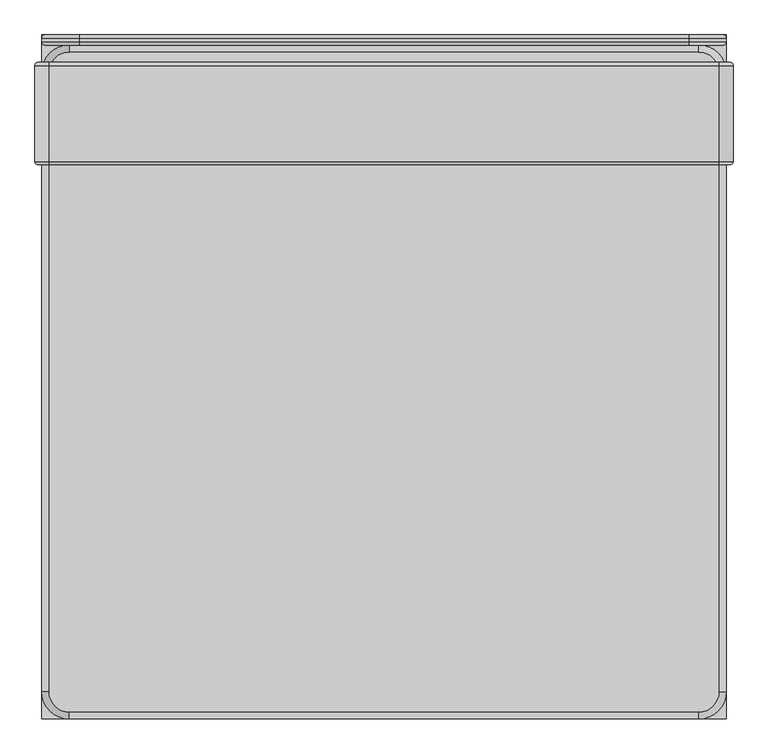
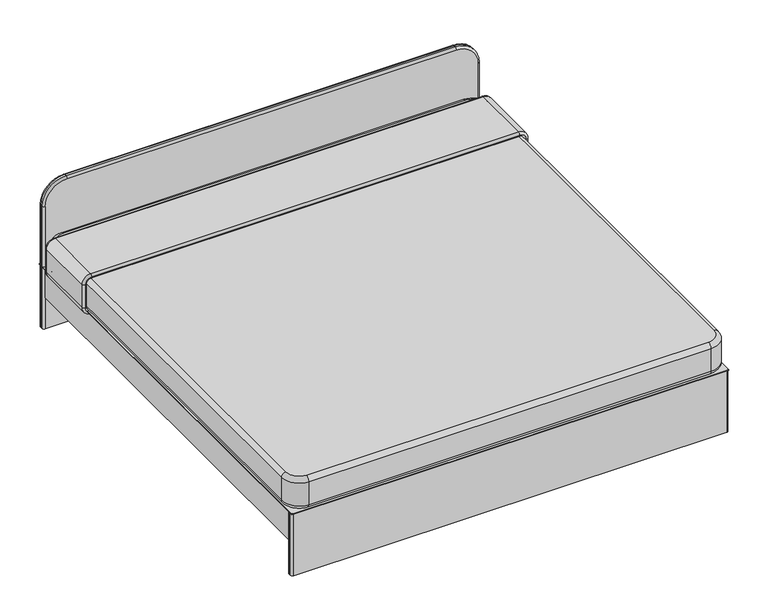
"""IFC4 building model written with IfcOpenShell, lengths in millimetres: furniture geometry, ベッド : 2000 x 2000 mm キング."""

from ifc_helpers import new_model, si_unit, point, frame, frame_2d, origin, origin_with_axes, place, context, project, spatial, polyline, circle_curve, ellipse_curve, trimmed, segment, composite_curve, outline, extrude, source, transform, mapped, element, save
from ifc_brep_helpers import plane_surface, cylinder_surface, revolved_surface, advanced_brep


def furniture_9038af62(model_context):
    return source(origin(), model_context, "Body", "SolidModel", [
        advanced_brep(
        [(1000.0, 960.0, 430.0), (1000.0, 680.0, 430.0), (980.0, 680.0, 450.0), (980.0, 960.0, 450.0), (1010.0, 970.0, 430.0), (980.0, 970.0, 460.0), (1020.0, 960.0, 430.0), (980.0, 960.0, 470.0), (1020.0, 680.0, 430.0), (980.0, 680.0, 470.0), (1010.0, 670.0, 430.0), (980.0, 670.0, 460.0), (1000.0, 960.0, 320.0), (1000.0, 680.0, 320.0), (1010.0, 970.0, 320.0), (1020.0, 960.0, 320.0), (1020.0, 680.0, 320.0), (1010.0, 670.0, 320.0), (980.0, 960.0, 300.0), (980.0, 680.0, 300.0), (980.0, 970.0, 290.0), (980.0, 960.0, 280.0), (980.0, 680.0, 280.0), (980.0, 670.0, 290.0), (-980.0, 960.0, 300.0), (-980.0, 680.0, 300.0), (-980.0, 970.0, 290.0), (-980.0, 960.0, 280.0), (-980.0, 680.0, 280.0), (-980.0, 670.0, 290.0), (-1000.0, 960.0, 320.0), (-1000.0, 680.0, 320.0), (-1010.0, 970.0, 320.0), (-1020.0, 960.0, 320.0), (-1020.0, 680.0, 320.0), (-1010.0, 670.0, 320.0), (-1000.0, 960.0, 430.0), (-1000.0, 680.0, 430.0), (-1010.0, 970.0, 430.0), (-1020.0, 960.0, 430.0), (-1020.0, 680.0, 430.0), (-1010.0, 670.0, 430.0), (-980.0, 960.0, 450.0), (-980.0, 680.0, 450.0), (-980.0, 970.0, 460.0), (-980.0, 960.0, 470.0), (-980.0, 680.0, 470.0), (-980.0, 670.0, 460.0)],
        [
            (0, 1),
            (1, 2, circle_curve(frame((980.0, 680.0, 430.0), z_axis=(0.0, -1.0, 0.0), x_axis=(0.0, 0.0, 1.0)), 20.0)),
            (2, 3),
            (3, 0, circle_curve(frame((980.0, 960.0, 430.0), z_axis=(0.0, 1.0, 0.0), x_axis=(0.0, 0.0, 1.0)), 20.0)),
            (4, 0, circle_curve(frame((1010.0, 960.0, 430.0), z_axis=(0.0, 0.0, 1.0), x_axis=(1.0, 0.0, 0.0)), 10.0)),
            (3, 5, circle_curve(frame((980.0, 960.0, 460.0), z_axis=(1.0, 0.0, 0.0), x_axis=(0.0, 0.0, 1.0)), 10.0)),
            (5, 4, circle_curve(frame((980.0, 970.0, 430.0), z_axis=(0.0, 1.0, 0.0), x_axis=(0.0, 0.0, 1.0)), 30.0)),
            (6, 4, circle_curve(frame((1010.0, 960.0, 430.0), z_axis=(0.0, 0.0, 1.0), x_axis=(1.0, 0.0, 0.0)), 10.0)),
            (5, 7, circle_curve(frame((980.0, 960.0, 460.0), z_axis=(1.0, 0.0, 0.0), x_axis=(0.0, 0.0, 1.0)), 10.0)),
            (7, 6, circle_curve(frame((980.0, 960.0, 430.0), z_axis=(0.0, 1.0, 0.0), x_axis=(0.0, 0.0, 1.0)), 40.0)),
            (8, 6),
            (7, 9),
            (9, 8, circle_curve(frame((980.0, 680.0, 430.0), z_axis=(0.0, 1.0, 0.0), x_axis=(0.0, 0.0, 1.0)), 40.0)),
            (10, 8, circle_curve(frame((1010.0, 680.0, 430.0), z_axis=(0.0, 0.0, 1.0), x_axis=(1.0, 0.0, 0.0)), 10.0)),
            (9, 11, circle_curve(frame((980.0, 680.0, 460.0), z_axis=(1.0, 0.0, 0.0), x_axis=(0.0, 0.0, 1.0)), 10.0)),
            (11, 10, circle_curve(frame((980.0, 670.0, 430.0), z_axis=(0.0, 1.0, 0.0), x_axis=(0.0, 0.0, 1.0)), 30.0)),
            (1, 10, circle_curve(frame((1010.0, 680.0, 430.0), z_axis=(0.0, 0.0, 1.0), x_axis=(1.0, 0.0, 0.0)), 10.0)),
            (11, 2, circle_curve(frame((980.0, 680.0, 460.0), z_axis=(1.0, 0.0, 0.0), x_axis=(0.0, 0.0, 1.0)), 10.0)),
            (0, 12),
            (12, 13),
            (13, 1),
            (4, 14),
            (14, 12, circle_curve(frame((1010.0, 960.0, 320.0), z_axis=(0.0, 0.0, 1.0), x_axis=(1.0, 0.0, 0.0)), 10.0)),
            (6, 15),
            (15, 14, circle_curve(frame((1010.0, 960.0, 320.0), z_axis=(0.0, 0.0, 1.0), x_axis=(1.0, 0.0, 0.0)), 10.0)),
            (8, 16),
            (16, 15),
            (10, 17),
            (17, 16, circle_curve(frame((1010.0, 680.0, 320.0), z_axis=(0.0, 0.0, 1.0), x_axis=(1.0, 0.0, 0.0)), 10.0)),
            (13, 17, circle_curve(frame((1010.0, 680.0, 320.0), z_axis=(0.0, 0.0, 1.0), x_axis=(1.0, 0.0, 0.0)), 10.0)),
            (18, 19),
            (19, 13, circle_curve(frame((980.0, 680.0, 320.0), z_axis=(0.0, -1.0, 0.0), x_axis=(1.0, 0.0, 0.0)), 20.0)),
            (12, 18, circle_curve(frame((980.0, 960.0, 320.0), z_axis=(0.0, 1.0, 0.0), x_axis=(1.0, 0.0, 0.0)), 20.0)),
            (20, 18, circle_curve(frame((980.0, 960.0, 290.0), z_axis=(1.0, 0.0, 0.0), x_axis=(0.0, 0.0, -1.0)), 10.0)),
            (14, 20, circle_curve(frame((980.0, 970.0, 320.0), z_axis=(0.0, 1.0, 0.0), x_axis=(1.0, 0.0, 0.0)), 30.0)),
            (21, 20, circle_curve(frame((980.0, 960.0, 290.0), z_axis=(1.0, 0.0, 0.0), x_axis=(0.0, 0.0, -1.0)), 10.0)),
            (15, 21, circle_curve(frame((980.0, 960.0, 320.0), z_axis=(0.0, 1.0, 0.0), x_axis=(1.0, 0.0, 0.0)), 40.0)),
            (22, 21),
            (16, 22, circle_curve(frame((980.0, 680.0, 320.0), z_axis=(0.0, 1.0, 0.0), x_axis=(1.0, 0.0, 0.0)), 40.0)),
            (23, 22, circle_curve(frame((980.0, 680.0, 290.0), z_axis=(1.0, 0.0, 0.0), x_axis=(0.0, 0.0, -1.0)), 10.0)),
            (17, 23, circle_curve(frame((980.0, 670.0, 320.0), z_axis=(0.0, 1.0, 0.0), x_axis=(1.0, 0.0, 0.0)), 30.0)),
            (19, 23, circle_curve(frame((980.0, 680.0, 290.0), z_axis=(1.0, 0.0, 0.0), x_axis=(0.0, 0.0, -1.0)), 10.0)),
            (18, 24),
            (24, 25),
            (25, 19),
            (20, 26),
            (26, 24, circle_curve(frame((-980.0, 960.0, 290.0), z_axis=(1.0, 0.0, 0.0), x_axis=(0.0, 0.0, -1.0)), 10.0)),
            (21, 27),
            (27, 26, circle_curve(frame((-980.0, 960.0, 290.0), z_axis=(1.0, 0.0, 0.0), x_axis=(0.0, 0.0, -1.0)), 10.0)),
            (22, 28),
            (28, 27),
            (23, 29),
            (29, 28, circle_curve(frame((-980.0, 680.0, 290.0), z_axis=(1.0, 0.0, 0.0), x_axis=(0.0, 0.0, -1.0)), 10.0)),
            (25, 29, circle_curve(frame((-980.0, 680.0, 290.0), z_axis=(1.0, 0.0, 0.0), x_axis=(0.0, 0.0, -1.0)), 10.0)),
            (30, 31),
            (31, 25, circle_curve(frame((-980.0, 680.0, 320.0), z_axis=(0.0, -1.0, 0.0), x_axis=(0.0, 0.0, -1.0)), 20.0)),
            (24, 30, circle_curve(frame((-980.0, 960.0, 320.0), z_axis=(0.0, 1.0, 0.0), x_axis=(0.0, 0.0, -1.0)), 20.0)),
            (32, 30, circle_curve(frame((-1010.0, 960.0, 320.0), z_axis=(0.0, 0.0, -1.0), x_axis=(-1.0, 0.0, 0.0)), 10.0)),
            (26, 32, circle_curve(frame((-980.0, 970.0, 320.0), z_axis=(0.0, 1.0, 0.0), x_axis=(0.0, 0.0, -1.0)), 30.0)),
            (33, 32, circle_curve(frame((-1010.0, 960.0, 320.0), z_axis=(0.0, 0.0, -1.0), x_axis=(-1.0, 0.0, 0.0)), 10.0)),
            (27, 33, circle_curve(frame((-980.0, 960.0, 320.0), z_axis=(0.0, 1.0, 0.0), x_axis=(0.0, 0.0, -1.0)), 40.0)),
            (34, 33),
            (28, 34, circle_curve(frame((-980.0, 680.0, 320.0), z_axis=(0.0, 1.0, 0.0), x_axis=(0.0, 0.0, -1.0)), 40.0)),
            (35, 34, circle_curve(frame((-1010.0, 680.0, 320.0), z_axis=(0.0, 0.0, -1.0), x_axis=(-1.0, 0.0, 0.0)), 10.0)),
            (29, 35, circle_curve(frame((-980.0, 670.0, 320.0), z_axis=(0.0, 1.0, 0.0), x_axis=(0.0, 0.0, -1.0)), 30.0)),
            (31, 35, circle_curve(frame((-1010.0, 680.0, 320.0), z_axis=(0.0, 0.0, -1.0), x_axis=(-1.0, 0.0, 0.0)), 10.0)),
            (30, 36),
            (36, 37),
            (37, 31),
            (32, 38),
            (38, 36, circle_curve(frame((-1010.0, 960.0, 430.0), z_axis=(0.0, 0.0, -1.0), x_axis=(-1.0, 0.0, 0.0)), 10.0)),
            (33, 39),
            (39, 38, circle_curve(frame((-1010.0, 960.0, 430.0), z_axis=(0.0, 0.0, -1.0), x_axis=(-1.0, 0.0, 0.0)), 10.0)),
            (34, 40),
            (40, 39),
            (35, 41),
            (41, 40, circle_curve(frame((-1010.0, 680.0, 430.0), z_axis=(0.0, 0.0, -1.0), x_axis=(-1.0, 0.0, 0.0)), 10.0)),
            (37, 41, circle_curve(frame((-1010.0, 680.0, 430.0), z_axis=(0.0, 0.0, -1.0), x_axis=(-1.0, 0.0, 0.0)), 10.0)),
            (42, 43),
            (43, 37, circle_curve(frame((-980.0, 680.0, 430.0), z_axis=(0.0, -1.0, 0.0), x_axis=(-1.0, 0.0, 0.0)), 20.0)),
            (36, 42, circle_curve(frame((-980.0, 960.0, 430.0), z_axis=(0.0, 1.0, 0.0), x_axis=(-1.0, 0.0, 0.0)), 20.0)),
            (44, 42, circle_curve(frame((-980.0, 960.0, 460.0), z_axis=(-1.0, 0.0, 0.0), x_axis=(0.0, 0.0, 1.0)), 10.0)),
            (38, 44, circle_curve(frame((-980.0, 970.0, 430.0), z_axis=(0.0, 1.0, 0.0), x_axis=(-1.0, 0.0, 0.0)), 30.0)),
            (45, 44, circle_curve(frame((-980.0, 960.0, 460.0), z_axis=(-1.0, 0.0, 0.0), x_axis=(0.0, 0.0, 1.0)), 10.0)),
            (39, 45, circle_curve(frame((-980.0, 960.0, 430.0), z_axis=(0.0, 1.0, 0.0), x_axis=(-1.0, 0.0, 0.0)), 40.0)),
            (46, 45),
            (40, 46, circle_curve(frame((-980.0, 680.0, 430.0), z_axis=(0.0, 1.0, 0.0), x_axis=(-1.0, 0.0, 0.0)), 40.0)),
            (47, 46, circle_curve(frame((-980.0, 680.0, 460.0), z_axis=(-1.0, 0.0, 0.0), x_axis=(0.0, 0.0, 1.0)), 10.0)),
            (41, 47, circle_curve(frame((-980.0, 670.0, 430.0), z_axis=(0.0, 1.0, 0.0), x_axis=(-1.0, 0.0, 0.0)), 30.0)),
            (43, 47, circle_curve(frame((-980.0, 680.0, 460.0), z_axis=(-1.0, 0.0, 0.0), x_axis=(0.0, 0.0, 1.0)), 10.0)),
            (42, 3),
            (2, 43),
            (44, 5),
            (45, 7),
            (46, 9),
            (47, 11),
        ],
        [
            revolved_surface(polyline([(980.0, 680.0, 450.0), (980.0, 960.0, 450.0)]), (980.0, 970.0, 430.0), (0.0, -1.0, 0.0)),
            revolved_surface(trimmed(ellipse_curve(frame((980.0, 960.0, 460.0), z_axis=(1.0, 0.0, 0.0), x_axis=(0.0, 0.0, 1.0)), 10.0, 10.0), [point((980.0, 960.0, 450.0))], [point((980.0, 970.0, 460.0))], True, "CARTESIAN"), (980.0, 970.0, 430.0), (0.0, -1.0, 0.0)),
            revolved_surface(trimmed(ellipse_curve(frame((980.0, 960.0, 460.0), z_axis=(1.0, 0.0, 0.0), x_axis=(0.0, 0.0, 1.0)), 10.0, 10.0), [point((980.0, 970.0, 460.0))], [point((980.0, 960.0, 470.0))], True, "CARTESIAN"), (980.0, 970.0, 430.0), (0.0, -1.0, 0.0)),
            cylinder_surface(frame((980.0, 970.0, 430.0), z_axis=(0.0, -1.0, 0.0), x_axis=(0.0, 0.0, 1.0)), 40.0),
            revolved_surface(trimmed(ellipse_curve(frame((980.0, 680.0, 460.0), z_axis=(1.0, 0.0, 0.0), x_axis=(0.0, 0.0, 1.0)), 10.0, 10.0), [point((980.0, 680.0, 470.0))], [point((980.0, 670.0, 460.0))], True, "CARTESIAN"), (980.0, 970.0, 430.0), (0.0, -1.0, 0.0)),
            revolved_surface(trimmed(ellipse_curve(frame((980.0, 680.0, 460.0), z_axis=(1.0, 0.0, 0.0), x_axis=(0.0, 0.0, 1.0)), 10.0, 10.0), [point((980.0, 670.0, 460.0))], [point((980.0, 680.0, 450.0))], True, "CARTESIAN"), (980.0, 970.0, 430.0), (0.0, -1.0, 0.0)),
            plane_surface(frame((1000.0, 680.0, 430.0), z_axis=(-1.0, 0.0, 0.0), x_axis=(0.0, 0.0, -1.0))),
            cylinder_surface(frame((1010.0, 960.0, 430.0), z_axis=(0.0, 0.0, 1.0), x_axis=(1.0, 0.0, 0.0)), 10.0),
            plane_surface(frame((1020.0, 960.0, 430.0), z_axis=(1.0, 0.0, 0.0), x_axis=(0.0, 0.0, -1.0))),
            cylinder_surface(frame((1010.0, 680.0, 430.0), z_axis=(0.0, 0.0, 1.0), x_axis=(1.0, 0.0, 0.0)), 10.0),
            revolved_surface(polyline([(1000.0, 680.0, 320.0), (1000.0, 960.0, 320.0)]), (980.0, 970.0, 320.0), (0.0, -1.0, 0.0)),
            revolved_surface(trimmed(ellipse_curve(frame((1010.0, 960.0, 320.0), z_axis=(0.0, 0.0, -1.0), x_axis=(1.0, 0.0, 0.0)), 10.0, 10.0), [point((1000.0, 960.0, 320.0))], [point((1010.0, 970.0, 320.0))], True, "CARTESIAN"), (980.0, 970.0, 320.0), (0.0, -1.0, 0.0)),
            revolved_surface(trimmed(ellipse_curve(frame((1010.0, 960.0, 320.0), z_axis=(0.0, 0.0, -1.0), x_axis=(1.0, 0.0, 0.0)), 10.0, 10.0), [point((1010.0, 970.0, 320.0))], [point((1020.0, 960.0, 320.0))], True, "CARTESIAN"), (980.0, 970.0, 320.0), (0.0, -1.0, 0.0)),
            cylinder_surface(frame((980.0, 970.0, 320.0), z_axis=(0.0, -1.0, 0.0), x_axis=(1.0, 0.0, 0.0)), 40.0),
            revolved_surface(trimmed(ellipse_curve(frame((1010.0, 680.0, 320.0), z_axis=(0.0, 0.0, -1.0), x_axis=(1.0, 0.0, 0.0)), 10.0, 10.0), [point((1020.0, 680.0, 320.0))], [point((1010.0, 670.0, 320.0))], True, "CARTESIAN"), (980.0, 970.0, 320.0), (0.0, -1.0, 0.0)),
            revolved_surface(trimmed(ellipse_curve(frame((1010.0, 680.0, 320.0), z_axis=(0.0, 0.0, -1.0), x_axis=(1.0, 0.0, 0.0)), 10.0, 10.0), [point((1010.0, 670.0, 320.0))], [point((1000.0, 680.0, 320.0))], True, "CARTESIAN"), (980.0, 970.0, 320.0), (0.0, -1.0, 0.0)),
            plane_surface(frame((980.0, 680.0, 300.0), z_axis=(0.0, 0.0, 1.0), x_axis=(-1.0, 0.0, 0.0))),
            cylinder_surface(frame((980.0, 960.0, 290.0), z_axis=(1.0, 0.0, 0.0), x_axis=(0.0, 0.0, -1.0)), 10.0),
            plane_surface(frame((980.0, 960.0, 280.0), z_axis=(0.0, 0.0, -1.0), x_axis=(-1.0, 0.0, 0.0))),
            cylinder_surface(frame((980.0, 680.0, 290.0), z_axis=(1.0, 0.0, 0.0), x_axis=(0.0, 0.0, -1.0)), 10.0),
            revolved_surface(polyline([(-980.0, 680.0, 300.0), (-980.0, 960.0, 300.0)]), (-980.0, 970.0, 320.0), (0.0, -1.0, 0.0)),
            revolved_surface(trimmed(ellipse_curve(frame((-980.0, 960.0, 290.0), z_axis=(-1.0, 0.0, 0.0), x_axis=(0.0, 0.0, -1.0)), 10.0, 10.0), [point((-980.0, 960.0, 300.0))], [point((-980.0, 970.0, 290.0))], True, "CARTESIAN"), (-980.0, 970.0, 320.0), (0.0, -1.0, 0.0)),
            revolved_surface(trimmed(ellipse_curve(frame((-980.0, 960.0, 290.0), z_axis=(-1.0, 0.0, 0.0), x_axis=(0.0, 0.0, -1.0)), 10.0, 10.0), [point((-980.0, 970.0, 290.0))], [point((-980.0, 960.0, 280.0))], True, "CARTESIAN"), (-980.0, 970.0, 320.0), (0.0, -1.0, 0.0)),
            cylinder_surface(frame((-980.0, 970.0, 320.0), z_axis=(0.0, -1.0, 0.0), x_axis=(0.0, 0.0, -1.0)), 40.0),
            revolved_surface(trimmed(ellipse_curve(frame((-980.0, 680.0, 290.0), z_axis=(-1.0, 0.0, 0.0), x_axis=(0.0, 0.0, -1.0)), 10.0, 10.0), [point((-980.0, 680.0, 280.0))], [point((-980.0, 670.0, 290.0))], True, "CARTESIAN"), (-980.0, 970.0, 320.0), (0.0, -1.0, 0.0)),
            revolved_surface(trimmed(ellipse_curve(frame((-980.0, 680.0, 290.0), z_axis=(-1.0, 0.0, 0.0), x_axis=(0.0, 0.0, -1.0)), 10.0, 10.0), [point((-980.0, 670.0, 290.0))], [point((-980.0, 680.0, 300.0))], True, "CARTESIAN"), (-980.0, 970.0, 320.0), (0.0, -1.0, 0.0)),
            plane_surface(frame((-1000.0, 680.0, 320.0), z_axis=(1.0, 0.0, 0.0), x_axis=(0.0, 0.0, 1.0))),
            cylinder_surface(frame((-1010.0, 960.0, 320.0), z_axis=(0.0, 0.0, -1.0), x_axis=(-1.0, 0.0, 0.0)), 10.0),
            plane_surface(frame((-1020.0, 960.0, 320.0), z_axis=(-1.0, 0.0, 0.0), x_axis=(0.0, 0.0, 1.0))),
            cylinder_surface(frame((-1010.0, 680.0, 320.0), z_axis=(0.0, 0.0, -1.0), x_axis=(-1.0, 0.0, 0.0)), 10.0),
            revolved_surface(polyline([(-1000.0, 680.0, 430.0), (-1000.0, 960.0, 430.0)]), (-980.0, 970.0, 430.0), (0.0, -1.0, 0.0)),
            revolved_surface(trimmed(ellipse_curve(frame((-1010.0, 960.0, 430.0), z_axis=(0.0, 0.0, 1.0), x_axis=(-1.0, 0.0, 0.0)), 10.0, 10.0), [point((-1000.0, 960.0, 430.0))], [point((-1010.0, 970.0, 430.0))], True, "CARTESIAN"), (-980.0, 970.0, 430.0), (0.0, -1.0, 0.0)),
            revolved_surface(trimmed(ellipse_curve(frame((-1010.0, 960.0, 430.0), z_axis=(0.0, 0.0, 1.0), x_axis=(-1.0, 0.0, 0.0)), 10.0, 10.0), [point((-1010.0, 970.0, 430.0))], [point((-1020.0, 960.0, 430.0))], True, "CARTESIAN"), (-980.0, 970.0, 430.0), (0.0, -1.0, 0.0)),
            cylinder_surface(frame((-980.0, 970.0, 430.0), z_axis=(0.0, -1.0, 0.0), x_axis=(-1.0, 0.0, 0.0)), 40.0),
            revolved_surface(trimmed(ellipse_curve(frame((-1010.0, 680.0, 430.0), z_axis=(0.0, 0.0, 1.0), x_axis=(-1.0, 0.0, 0.0)), 10.0, 10.0), [point((-1020.0, 680.0, 430.0))], [point((-1010.0, 670.0, 430.0))], True, "CARTESIAN"), (-980.0, 970.0, 430.0), (0.0, -1.0, 0.0)),
            revolved_surface(trimmed(ellipse_curve(frame((-1010.0, 680.0, 430.0), z_axis=(0.0, 0.0, 1.0), x_axis=(-1.0, 0.0, 0.0)), 10.0, 10.0), [point((-1010.0, 670.0, 430.0))], [point((-1000.0, 680.0, 430.0))], True, "CARTESIAN"), (-980.0, 970.0, 430.0), (0.0, -1.0, 0.0)),
            plane_surface(frame((-980.0, 680.0, 450.0), z_axis=(0.0, 0.0, -1.0), x_axis=(1.0, 0.0, 0.0))),
            cylinder_surface(frame((-980.0, 960.0, 460.0), z_axis=(-1.0, 0.0, 0.0), x_axis=(0.0, 0.0, 1.0)), 10.0),
            plane_surface(frame((-980.0, 960.0, 470.0), z_axis=(0.0, 0.0, 1.0), x_axis=(1.0, 0.0, 0.0))),
            cylinder_surface(frame((-980.0, 680.0, 460.0), z_axis=(-1.0, 0.0, 0.0), x_axis=(0.0, 0.0, 1.0)), 10.0),
        ],
        [
            (0, [[1, 2, 3, 4]]),
            (1, [[5, -4, 6, 7]]),
            (2, [[8, -7, 9, 10]]),
            (3, [[11, -10, 12, 13]]),
            (4, [[14, -13, 15, 16]]),
            (5, [[17, -16, 18, -2]]),
            (6, [[19, 20, 21, -1]]),
            (7, [[22, 23, -19, -5]]),
            (7, [[24, 25, -22, -8]]),
            (8, [[26, 27, -24, -11]]),
            (9, [[28, 29, -26, -14]]),
            (9, [[-21, 30, -28, -17]]),
            (10, [[31, 32, -20, 33]]),
            (11, [[34, -33, -23, 35]]),
            (12, [[36, -35, -25, 37]]),
            (13, [[38, -37, -27, 39]]),
            (14, [[40, -39, -29, 41]]),
            (15, [[42, -41, -30, -32]]),
            (16, [[43, 44, 45, -31]]),
            (17, [[46, 47, -43, -34]]),
            (17, [[48, 49, -46, -36]]),
            (18, [[50, 51, -48, -38]]),
            (19, [[52, 53, -50, -40]]),
            (19, [[-45, 54, -52, -42]]),
            (20, [[55, 56, -44, 57]]),
            (21, [[58, -57, -47, 59]]),
            (22, [[60, -59, -49, 61]]),
            (23, [[62, -61, -51, 63]]),
            (24, [[64, -63, -53, 65]]),
            (25, [[66, -65, -54, -56]]),
            (26, [[67, 68, 69, -55]]),
            (27, [[70, 71, -67, -58]]),
            (27, [[72, 73, -70, -60]]),
            (28, [[74, 75, -72, -62]]),
            (29, [[76, 77, -74, -64]]),
            (29, [[-69, 78, -76, -66]]),
            (30, [[79, 80, -68, 81]]),
            (31, [[82, -81, -71, 83]]),
            (32, [[84, -83, -73, 85]]),
            (33, [[86, -85, -75, 87]]),
            (34, [[88, -87, -77, 89]]),
            (35, [[90, -89, -78, -80]]),
            (36, [[91, -3, 92, -79]]),
            (37, [[93, -6, -91, -82]]),
            (37, [[94, -9, -93, -84]]),
            (38, [[95, -12, -94, -86]]),
            (39, [[96, -15, -95, -88]]),
            (39, [[-92, -18, -96, -90]]),
        ],
    ),
        extrude(outline(polyline([(1000.0, 1050.0), (1000.0, -950.0), (-1000.0, -950.0), (-1000.0, 1050.0), (1000.0, 1050.0)])), frame((0.0, 0.0, 298.0), z_axis=(0.0, 0.0, 1.0), x_axis=(1.0, 0.0, 0.0)), (0.0, 0.0, 1.0), 2.0),
        advanced_brep(
        [(1000.0, 940.0, 320.0), (980.0, 940.0, 300.0), (920.0, 1000.0, 300.0), (920.0, 1020.0, 320.0), (920.0, 1020.0, 430.0), (1000.0, 940.0, 430.0), (920.0, 1000.0, 450.0), (980.0, 940.0, 450.0), (1000.0, -870.0, 320.0), (980.0, -870.0, 300.0), (1000.0, -870.0, 430.0), (980.0, -870.0, 450.0), (920.0, -950.0, 320.0), (920.0, -930.0, 300.0), (920.0, -950.0, 430.0), (920.0, -930.0, 450.0), (-920.0, -950.0, 320.0), (-920.0, -930.0, 300.0), (-920.0, -950.0, 430.0), (-920.0, -930.0, 450.0), (-1000.0, -870.0, 320.0), (-980.0, -870.0, 300.0), (-1000.0, -870.0, 430.0), (-980.0, -870.0, 450.0), (-1000.0, 940.0, 320.0), (-980.0, 940.0, 300.0), (-1000.0, 940.0, 430.0), (-980.0, 940.0, 450.0), (-920.0, 1020.0, 320.0), (-920.0, 1000.0, 300.0), (-920.0, 1020.0, 430.0), (-920.0, 1000.0, 450.0)],
        [
            (0, 1, circle_curve(frame((980.0, 940.0, 320.0), z_axis=(0.0, 1.0, 0.0), x_axis=(-1.0, 0.0, 0.0)), 20.0)),
            (1, 2, circle_curve(frame((920.0, 940.0, 300.0), z_axis=(0.0, 0.0, 1.0), x_axis=(0.0, 1.0, 0.0)), 60.0)),
            (2, 3, circle_curve(frame((920.0, 1000.0, 320.0), z_axis=(1.0, 0.0, 0.0), x_axis=(0.0, -1.0, 0.0)), 20.0)),
            (3, 0, circle_curve(frame((920.0, 940.0, 320.0), z_axis=(0.0, 0.0, -1.0), x_axis=(0.0, 1.0, 0.0)), 80.0)),
            (3, 4),
            (4, 5, circle_curve(frame((920.0, 940.0, 430.0), z_axis=(0.0, 0.0, -1.0), x_axis=(0.0, 1.0, 0.0)), 80.0)),
            (5, 0),
            (4, 6, circle_curve(frame((920.0, 1000.0, 430.0), z_axis=(1.0, 0.0, 0.0), x_axis=(0.0, -1.0, 0.0)), 20.0)),
            (6, 7, circle_curve(frame((920.0, 940.0, 450.0), z_axis=(0.0, 0.0, -1.0), x_axis=(0.0, 1.0, 0.0)), 60.0)),
            (7, 5, circle_curve(frame((980.0, 940.0, 430.0), z_axis=(0.0, 1.0, 0.0), x_axis=(-1.0, 0.0, 0.0)), 20.0)),
            (0, 8),
            (8, 9, circle_curve(frame((980.0, -870.0, 320.0), z_axis=(0.0, 1.0, 0.0), x_axis=(-1.0, 0.0, 0.0)), 20.0)),
            (9, 1),
            (5, 10),
            (10, 8),
            (7, 11),
            (11, 10, circle_curve(frame((980.0, -870.0, 430.0), z_axis=(0.0, 1.0, 0.0), x_axis=(-1.0, 0.0, 0.0)), 20.0)),
            (8, 12, circle_curve(frame((920.0, -870.0, 320.0), z_axis=(0.0, 0.0, -1.0), x_axis=(1.0, 0.0, 0.0)), 80.0)),
            (12, 13, circle_curve(frame((920.0, -930.0, 320.0), z_axis=(1.0, 0.0, 0.0), x_axis=(0.0, 1.0, 0.0)), 20.0)),
            (13, 9, circle_curve(frame((920.0, -870.0, 300.0), z_axis=(0.0, 0.0, 1.0), x_axis=(1.0, 0.0, 0.0)), 60.0)),
            (10, 14, circle_curve(frame((920.0, -870.0, 430.0), z_axis=(0.0, 0.0, -1.0), x_axis=(1.0, 0.0, 0.0)), 80.0)),
            (14, 12),
            (11, 15, circle_curve(frame((920.0, -870.0, 450.0), z_axis=(0.0, 0.0, -1.0), x_axis=(1.0, 0.0, 0.0)), 60.0)),
            (15, 14, circle_curve(frame((920.0, -930.0, 430.0), z_axis=(1.0, 0.0, 0.0), x_axis=(0.0, 1.0, 0.0)), 20.0)),
            (12, 16),
            (16, 17, circle_curve(frame((-920.0, -930.0, 320.0), z_axis=(1.0, 0.0, 0.0), x_axis=(0.0, 1.0, 0.0)), 20.0)),
            (17, 13),
            (14, 18),
            (18, 16),
            (15, 19),
            (19, 18, circle_curve(frame((-920.0, -930.0, 430.0), z_axis=(1.0, 0.0, 0.0), x_axis=(0.0, 1.0, 0.0)), 20.0)),
            (16, 20, circle_curve(frame((-920.0, -870.0, 320.0), z_axis=(0.0, 0.0, -1.0), x_axis=(0.0, -1.0, 0.0)), 80.0)),
            (20, 21, circle_curve(frame((-980.0, -870.0, 320.0), z_axis=(0.0, -1.0, 0.0), x_axis=(1.0, 0.0, 0.0)), 20.0)),
            (21, 17, circle_curve(frame((-920.0, -870.0, 300.0), z_axis=(0.0, 0.0, 1.0), x_axis=(0.0, -1.0, 0.0)), 60.0)),
            (18, 22, circle_curve(frame((-920.0, -870.0, 430.0), z_axis=(0.0, 0.0, -1.0), x_axis=(0.0, -1.0, 0.0)), 80.0)),
            (22, 20),
            (19, 23, circle_curve(frame((-920.0, -870.0, 450.0), z_axis=(0.0, 0.0, -1.0), x_axis=(0.0, -1.0, 0.0)), 60.0)),
            (23, 22, circle_curve(frame((-980.0, -870.0, 430.0), z_axis=(0.0, -1.0, 0.0), x_axis=(1.0, 0.0, 0.0)), 20.0)),
            (20, 24),
            (24, 25, circle_curve(frame((-980.0, 940.0, 320.0), z_axis=(0.0, -1.0, 0.0), x_axis=(1.0, 0.0, 0.0)), 20.0)),
            (25, 21),
            (22, 26),
            (26, 24),
            (23, 27),
            (27, 26, circle_curve(frame((-980.0, 940.0, 430.0), z_axis=(0.0, -1.0, 0.0), x_axis=(1.0, 0.0, 0.0)), 20.0)),
            (24, 28, circle_curve(frame((-920.0, 940.0, 320.0), z_axis=(0.0, 0.0, -1.0), x_axis=(-1.0, 0.0, 0.0)), 80.0)),
            (28, 29, circle_curve(frame((-920.0, 1000.0, 320.0), z_axis=(-1.0, 0.0, 0.0), x_axis=(0.0, -1.0, 0.0)), 20.0)),
            (29, 25, circle_curve(frame((-920.0, 940.0, 300.0), z_axis=(0.0, 0.0, 1.0), x_axis=(-1.0, 0.0, 0.0)), 60.0)),
            (26, 30, circle_curve(frame((-920.0, 940.0, 430.0), z_axis=(0.0, 0.0, -1.0), x_axis=(-1.0, 0.0, 0.0)), 80.0)),
            (30, 28),
            (27, 31, circle_curve(frame((-920.0, 940.0, 450.0), z_axis=(0.0, 0.0, -1.0), x_axis=(-1.0, 0.0, 0.0)), 60.0)),
            (31, 30, circle_curve(frame((-920.0, 1000.0, 430.0), z_axis=(-1.0, 0.0, 0.0), x_axis=(0.0, -1.0, 0.0)), 20.0)),
            (6, 31),
            (29, 2),
            (28, 3),
            (30, 4),
        ],
        [
            revolved_surface(trimmed(ellipse_curve(frame((920.0, 1000.0, 320.0), z_axis=(1.0, 0.0, 0.0), x_axis=(0.0, -1.0, 0.0)), 20.0, 20.0), [point((920.0, 1000.0, 300.0))], [point((920.0, 1020.0, 320.0))], True, "CARTESIAN"), (920.0, 940.0, 300.0), (0.0, 0.0, 1.0)),
            cylinder_surface(frame((920.0, 940.0, 300.0), z_axis=(0.0, 0.0, 1.0), x_axis=(0.0, 1.0, 0.0)), 80.0),
            revolved_surface(trimmed(ellipse_curve(frame((920.0, 1000.0, 430.0), z_axis=(1.0, 0.0, 0.0), x_axis=(0.0, -1.0, 0.0)), 20.0, 20.0), [point((920.0, 1020.0, 430.0))], [point((920.0, 1000.0, 450.0))], True, "CARTESIAN"), (920.0, 940.0, 300.0), (0.0, 0.0, 1.0)),
            cylinder_surface(frame((980.0, 940.0, 320.0), z_axis=(0.0, 1.0, 0.0), x_axis=(-1.0, 0.0, 0.0)), 20.0),
            plane_surface(frame((1000.0, 940.0, 320.0), z_axis=(1.0, 0.0, 0.0), x_axis=(0.0, -1.0, 0.0))),
            cylinder_surface(frame((980.0, 940.0, 430.0), z_axis=(0.0, 1.0, 0.0), x_axis=(-1.0, 0.0, 0.0)), 20.0),
            revolved_surface(trimmed(ellipse_curve(frame((980.0, -870.0, 320.0), z_axis=(0.0, -1.0, 0.0), x_axis=(-1.0, 0.0, 0.0)), 20.0, 20.0), [point((980.0, -870.0, 300.0))], [point((1000.0, -870.0, 320.0))], True, "CARTESIAN"), (920.0, -870.0, 300.0), (0.0, 0.0, 1.0)),
            cylinder_surface(frame((920.0, -870.0, 300.0), z_axis=(0.0, 0.0, 1.0), x_axis=(1.0, 0.0, 0.0)), 80.0),
            revolved_surface(trimmed(ellipse_curve(frame((980.0, -870.0, 430.0), z_axis=(0.0, -1.0, 0.0), x_axis=(-1.0, 0.0, 0.0)), 20.0, 20.0), [point((1000.0, -870.0, 430.0))], [point((980.0, -870.0, 450.0))], True, "CARTESIAN"), (920.0, -870.0, 300.0), (0.0, 0.0, 1.0)),
            cylinder_surface(frame((920.0, -930.0, 320.0), z_axis=(1.0, 0.0, 0.0), x_axis=(0.0, 1.0, 0.0)), 20.0),
            plane_surface(frame((920.0, -950.0, 320.0), z_axis=(0.0, -1.0, 0.0), x_axis=(-1.0, 0.0, 0.0))),
            cylinder_surface(frame((920.0, -930.0, 430.0), z_axis=(1.0, 0.0, 0.0), x_axis=(0.0, 1.0, 0.0)), 20.0),
            revolved_surface(trimmed(ellipse_curve(frame((-920.0, -930.0, 320.0), z_axis=(-1.0, 0.0, 0.0), x_axis=(0.0, 1.0, 0.0)), 20.0, 20.0), [point((-920.0, -930.0, 300.0))], [point((-920.0, -950.0, 320.0))], True, "CARTESIAN"), (-920.0, -870.0, 300.0), (0.0, 0.0, 1.0)),
            cylinder_surface(frame((-920.0, -870.0, 300.0), z_axis=(0.0, 0.0, 1.0), x_axis=(0.0, -1.0, 0.0)), 80.0),
            revolved_surface(trimmed(ellipse_curve(frame((-920.0, -930.0, 430.0), z_axis=(-1.0, 0.0, 0.0), x_axis=(0.0, 1.0, 0.0)), 20.0, 20.0), [point((-920.0, -950.0, 430.0))], [point((-920.0, -930.0, 450.0))], True, "CARTESIAN"), (-920.0, -870.0, 300.0), (0.0, 0.0, 1.0)),
            cylinder_surface(frame((-980.0, -870.0, 320.0), z_axis=(0.0, -1.0, 0.0), x_axis=(1.0, 0.0, 0.0)), 20.0),
            plane_surface(frame((-1000.0, -870.0, 320.0), z_axis=(-1.0, 0.0, 0.0), x_axis=(0.0, 1.0, 0.0))),
            cylinder_surface(frame((-980.0, -870.0, 430.0), z_axis=(0.0, -1.0, 0.0), x_axis=(1.0, 0.0, 0.0)), 20.0),
            revolved_surface(trimmed(ellipse_curve(frame((-980.0, 940.0, 320.0), z_axis=(0.0, 1.0, 0.0), x_axis=(1.0, 0.0, 0.0)), 20.0, 20.0), [point((-980.0, 940.0, 300.0))], [point((-1000.0, 940.0, 320.0))], True, "CARTESIAN"), (-920.0, 940.0, 300.0), (0.0, 0.0, 1.0)),
            cylinder_surface(frame((-920.0, 940.0, 300.0), z_axis=(0.0, 0.0, 1.0), x_axis=(-1.0, 0.0, 0.0)), 80.0),
            revolved_surface(trimmed(ellipse_curve(frame((-980.0, 940.0, 430.0), z_axis=(0.0, 1.0, 0.0), x_axis=(1.0, 0.0, 0.0)), 20.0, 20.0), [point((-1000.0, 940.0, 430.0))], [point((-980.0, 940.0, 450.0))], True, "CARTESIAN"), (-920.0, 940.0, 300.0), (0.0, 0.0, 1.0)),
            plane_surface(frame((-920.0, 940.0, 450.0), z_axis=(0.0, 0.0, 1.0), x_axis=(-1.0, 0.0, 0.0))),
            plane_surface(frame((-920.0, 940.0, 300.0), z_axis=(0.0, 0.0, -1.0), x_axis=(-1.0, 0.0, 0.0))),
            cylinder_surface(frame((-920.0, 1000.0, 320.0), z_axis=(-1.0, 0.0, 0.0), x_axis=(0.0, -1.0, 0.0)), 20.0),
            plane_surface(frame((-920.0, 1020.0, 320.0), z_axis=(0.0, 1.0, 0.0), x_axis=(1.0, 0.0, 0.0))),
            cylinder_surface(frame((-920.0, 1000.0, 430.0), z_axis=(-1.0, 0.0, 0.0), x_axis=(0.0, -1.0, 0.0)), 20.0),
        ],
        [
            (0, [[1, 2, 3, 4]]),
            (1, [[5, 6, 7, -4]]),
            (2, [[8, 9, 10, -6]]),
            (3, [[11, 12, 13, -1]]),
            (4, [[14, 15, -11, -7]]),
            (5, [[16, 17, -14, -10]]),
            (6, [[18, 19, 20, -12]]),
            (7, [[21, 22, -18, -15]]),
            (8, [[23, 24, -21, -17]]),
            (9, [[25, 26, 27, -19]]),
            (10, [[28, 29, -25, -22]]),
            (11, [[30, 31, -28, -24]]),
            (12, [[32, 33, 34, -26]]),
            (13, [[35, 36, -32, -29]]),
            (14, [[37, 38, -35, -31]]),
            (15, [[39, 40, 41, -33]]),
            (16, [[42, 43, -39, -36]]),
            (17, [[44, 45, -42, -38]]),
            (18, [[46, 47, 48, -40]]),
            (19, [[49, 50, -46, -43]]),
            (20, [[51, 52, -49, -45]]),
            (21, [[53, -51, -44, -37, -30, -23, -16, -9]]),
            (22, [[-13, -20, -27, -34, -41, -48, 54, -2]]),
            (23, [[-54, -47, 55, -3]]),
            (24, [[-55, -50, 56, -5]]),
            (25, [[-56, -52, -53, -8]]),
        ],
    ),
        extrude(outline(polyline([(990.0, 1020.0), (990.0, -920.0), (-990.0, -920.0), (-990.0, 1020.0), (990.0, 1020.0)])), frame((0.0, 0.0, 150.0), z_axis=(0.0, 0.0, 1.0), x_axis=(1.0, 0.0, 0.0)), (0.0, 0.0, 1.0), 150.0),
        extrude(outline(composite_curve([segment(polyline([(990.0, -950.0), (-990.0, -950.0)]), True, "CONTINUOUS"), segment(trimmed(circle_curve(frame_2d((-990.0, -940.0)), 10.0), [point((-990.0, -950.0))], [point((-1000.0, -940.0))], False, "CARTESIAN"), True, "CONTINUOUS"), segment(polyline([(-1000.0, -940.0), (-1000.0, -930.0)]), True, "CONTINUOUS"), segment(trimmed(circle_curve(frame_2d((-990.0, -930.0)), 10.0), [point((-1000.0, -930.0))], [point((-990.0, -920.0))], False, "CARTESIAN"), True, "CONTINUOUS"), segment(polyline([(-990.0, -920.0), (990.0, -920.0)]), True, "CONTINUOUS"), segment(trimmed(circle_curve(frame_2d((990.0, -930.0)), 10.0), [point((990.0, -920.0))], [point((1000.0, -930.0))], False, "CARTESIAN"), True, "CONTINUOUS"), segment(polyline([(1000.0, -930.0), (1000.0, -940.0)]), True, "CONTINUOUS"), segment(trimmed(circle_curve(frame_2d((990.0, -940.0)), 10.0), [point((1000.0, -940.0))], [point((990.0, -950.0))], False, "CARTESIAN"), True, "CONTINUOUS")], self_intersect=False)), origin_with_axes(), (0.0, 0.0, 1.0), 300.0),
        advanced_brep(
        [(-990.0, 1050.0, 0.0), (990.0, 1050.0, 0.0), (1000.0, 1040.0, 0.0), (1000.0, 1030.0, 0.0), (990.0, 1020.0, 0.0), (-990.0, 1020.0, 0.0), (-1000.0, 1030.0, 0.0), (-1000.0, 1040.0, 0.0), (-990.0, 1050.0, 590.0), (-890.0, 1050.0, 690.0), (890.0, 1050.0, 690.0), (990.0, 1050.0, 590.0), (-1000.0, 1040.0, 590.0), (-1000.0, 1030.0, 590.0), (-990.0, 1020.0, 590.0), (990.0, 1020.0, 590.0), (890.0, 1020.0, 690.0), (-890.0, 1020.0, 690.0), (-890.0, 1040.0, 700.0), (-890.0, 1030.0, 700.0), (890.0, 1040.0, 700.0), (890.0, 1030.0, 700.0), (1000.0, 1040.0, 590.0), (1000.0, 1030.0, 590.0)],
        [
            (0, 1),
            (1, 2, circle_curve(frame((990.0, 1040.0, 0.0), z_axis=(0.0, 0.0, -1.0), x_axis=(1.0, 0.0, 0.0)), 10.0)),
            (2, 3),
            (3, 4, circle_curve(frame((990.0, 1030.0, 0.0), z_axis=(0.0, 0.0, -1.0), x_axis=(1.0, 0.0, 0.0)), 10.0)),
            (4, 5),
            (5, 6, circle_curve(frame((-990.0, 1030.0, 0.0), z_axis=(0.0, 0.0, -1.0), x_axis=(-1.0, 0.0, 0.0)), 10.0)),
            (6, 7),
            (7, 0, circle_curve(frame((-990.0, 1040.0, 0.0), z_axis=(0.0, 0.0, -1.0), x_axis=(-1.0, 0.0, 0.0)), 10.0)),
            (0, 8),
            (8, 9, circle_curve(frame((-890.0, 1050.0, 590.0), z_axis=(0.0, 1.0, 0.0), x_axis=(-1.0, 0.0, 0.0)), 100.0)),
            (9, 10),
            (10, 11, circle_curve(frame((890.0, 1050.0, 590.0), z_axis=(0.0, 1.0, 0.0), x_axis=(0.0, 0.0, 1.0)), 100.0)),
            (11, 1),
            (7, 12),
            (12, 8, circle_curve(frame((-990.0, 1040.0, 590.0), z_axis=(0.0, 0.0, -1.0), x_axis=(-1.0, 0.0, 0.0)), 10.0)),
            (6, 13),
            (13, 12),
            (5, 14),
            (14, 13, circle_curve(frame((-990.0, 1030.0, 590.0), z_axis=(0.0, 0.0, -1.0), x_axis=(-1.0, 0.0, 0.0)), 10.0)),
            (4, 15),
            (15, 16, circle_curve(frame((890.0, 1020.0, 590.0), z_axis=(0.0, -1.0, 0.0), x_axis=(0.0, 0.0, 1.0)), 100.0)),
            (16, 17),
            (17, 14, circle_curve(frame((-890.0, 1020.0, 590.0), z_axis=(0.0, -1.0, 0.0), x_axis=(-1.0, 0.0, 0.0)), 100.0)),
            (12, 18, circle_curve(frame((-890.0, 1040.0, 590.0), z_axis=(0.0, 1.0, 0.0), x_axis=(-1.0, 0.0, 0.0)), 110.0)),
            (18, 9, circle_curve(frame((-890.0, 1040.0, 690.0), z_axis=(-1.0, 0.0, 0.0), x_axis=(0.0, 0.0, 1.0)), 10.0)),
            (13, 19, circle_curve(frame((-890.0, 1030.0, 590.0), z_axis=(0.0, 1.0, 0.0), x_axis=(-1.0, 0.0, 0.0)), 110.0)),
            (19, 18),
            (17, 19, circle_curve(frame((-890.0, 1030.0, 690.0), z_axis=(-1.0, 0.0, 0.0), x_axis=(0.0, 0.0, 1.0)), 10.0)),
            (18, 20),
            (20, 10, circle_curve(frame((890.0, 1040.0, 690.0), z_axis=(-1.0, 0.0, 0.0), x_axis=(0.0, 0.0, 1.0)), 10.0)),
            (19, 21),
            (21, 20),
            (16, 21, circle_curve(frame((890.0, 1030.0, 690.0), z_axis=(-1.0, 0.0, 0.0), x_axis=(0.0, 0.0, 1.0)), 10.0)),
            (20, 22, circle_curve(frame((890.0, 1040.0, 590.0), z_axis=(0.0, 1.0, 0.0), x_axis=(0.0, 0.0, 1.0)), 110.0)),
            (22, 11, circle_curve(frame((990.0, 1040.0, 590.0), z_axis=(0.0, 0.0, 1.0), x_axis=(1.0, 0.0, 0.0)), 10.0)),
            (21, 23, circle_curve(frame((890.0, 1030.0, 590.0), z_axis=(0.0, 1.0, 0.0), x_axis=(0.0, 0.0, 1.0)), 110.0)),
            (23, 22),
            (15, 23, circle_curve(frame((990.0, 1030.0, 590.0), z_axis=(0.0, 0.0, 1.0), x_axis=(1.0, 0.0, 0.0)), 10.0)),
            (22, 2),
            (23, 3),
        ],
        [
            plane_surface(frame((-940.0, 1113.2455532, 0.0), z_axis=(0.0, 0.0, -1.0), x_axis=(1.0, 0.0, 0.0))),
            plane_surface(frame((-940.0, 1050.0, 0.0), z_axis=(0.0, 1.0, 0.0), x_axis=(0.0, 0.0, 1.0))),
            cylinder_surface(frame((-990.0, 1040.0, 0.0), z_axis=(0.0, 0.0, -1.0), x_axis=(-1.0, 0.0, 0.0)), 10.0),
            plane_surface(frame((-1000.0, 1040.0, 0.0), z_axis=(-1.0, 0.0, 0.0), x_axis=(0.0, 0.0, 1.0))),
            cylinder_surface(frame((-990.0, 1030.0, 0.0), z_axis=(0.0, 0.0, -1.0), x_axis=(-1.0, 0.0, 0.0)), 10.0),
            plane_surface(frame((-990.0, 1020.0, 0.0), z_axis=(0.0, -1.0, 0.0), x_axis=(0.0, 0.0, 1.0))),
            revolved_surface(trimmed(ellipse_curve(frame((-990.0, 1040.0, 590.0), z_axis=(0.0, 0.0, 1.0), x_axis=(-1.0, 0.0, 0.0)), 10.0, 10.0), [point((-990.0, 1050.0, 590.0))], [point((-1000.0, 1040.0, 590.0))], True, "CARTESIAN"), (-890.0, 1050.0, 590.0), (0.0, -1.0, 0.0)),
            cylinder_surface(frame((-890.0, 1050.0, 590.0), z_axis=(0.0, -1.0, 0.0), x_axis=(-1.0, 0.0, 0.0)), 110.0),
            revolved_surface(trimmed(ellipse_curve(frame((-990.0, 1030.0, 590.0), z_axis=(0.0, 0.0, 1.0), x_axis=(-1.0, 0.0, 0.0)), 10.0, 10.0), [point((-1000.0, 1030.0, 590.0))], [point((-990.0, 1020.0, 590.0))], True, "CARTESIAN"), (-890.0, 1050.0, 590.0), (0.0, -1.0, 0.0)),
            cylinder_surface(frame((-890.0, 1040.0, 690.0), z_axis=(-1.0, 0.0, 0.0), x_axis=(0.0, 0.0, 1.0)), 10.0),
            plane_surface(frame((-890.0, 1040.0, 700.0), z_axis=(0.0, 0.0, 1.0), x_axis=(1.0, 0.0, 0.0))),
            cylinder_surface(frame((-890.0, 1030.0, 690.0), z_axis=(-1.0, 0.0, 0.0), x_axis=(0.0, 0.0, 1.0)), 10.0),
            revolved_surface(trimmed(ellipse_curve(frame((890.0, 1040.0, 690.0), z_axis=(1.0, 0.0, 0.0), x_axis=(0.0, 0.0, 1.0)), 10.0, 10.0), [point((890.0, 1050.0, 690.0))], [point((890.0, 1040.0, 700.0))], True, "CARTESIAN"), (890.0, 1050.0, 590.0), (0.0, -1.0, 0.0)),
            cylinder_surface(frame((890.0, 1050.0, 590.0), z_axis=(0.0, -1.0, 0.0), x_axis=(0.0, 0.0, 1.0)), 110.0),
            revolved_surface(trimmed(ellipse_curve(frame((890.0, 1030.0, 690.0), z_axis=(1.0, 0.0, 0.0), x_axis=(0.0, 0.0, 1.0)), 10.0, 10.0), [point((890.0, 1030.0, 700.0))], [point((890.0, 1020.0, 690.0))], True, "CARTESIAN"), (890.0, 1050.0, 590.0), (0.0, -1.0, 0.0)),
            cylinder_surface(frame((990.0, 1040.0, 590.0), z_axis=(0.0, 0.0, 1.0), x_axis=(1.0, 0.0, 0.0)), 10.0),
            plane_surface(frame((1000.0, 1040.0, 590.0), z_axis=(1.0, 0.0, 0.0), x_axis=(0.0, 0.0, -1.0))),
            cylinder_surface(frame((990.0, 1030.0, 590.0), z_axis=(0.0, 0.0, 1.0), x_axis=(1.0, 0.0, 0.0)), 10.0),
        ],
        [
            (0, [[1, 2, 3, 4, 5, 6, 7, 8]]),
            (1, [[9, 10, 11, 12, 13, -1]]),
            (2, [[14, 15, -9, -8]]),
            (3, [[16, 17, -14, -7]]),
            (4, [[18, 19, -16, -6]]),
            (5, [[20, 21, 22, 23, -18, -5]]),
            (6, [[-15, 24, 25, -10]]),
            (7, [[26, 27, -24, -17]]),
            (8, [[-23, 28, -26, -19]]),
            (9, [[-25, 29, 30, -11]]),
            (10, [[31, 32, -29, -27]]),
            (11, [[33, -31, -28, -22]]),
            (12, [[-30, 34, 35, -12]]),
            (13, [[36, 37, -34, -32]]),
            (14, [[38, -36, -33, -21]]),
            (15, [[-35, 39, -2, -13]]),
            (16, [[40, -3, -39, -37]]),
            (17, [[-4, -40, -38, -20]]),
        ],
    ),
    ])


if __name__ == "__main__":
    model = new_model("IFC4")
    model_context = context("Model", 3, world=origin())
    ifc_project = project(units=[si_unit("LENGTHUNIT", "METRE", prefix="MILLI")], contexts=[model_context])
    site = spatial("IfcSite", under=ifc_project)
    building = spatial("IfcBuilding", under=site)
    placement = place(None, origin())
    furniture_shape = furniture_9038af62(model_context)
    element("IfcFurniture", 1, ObjectType="ベッド : 2000 x 2000 mm キング", at=placement, inside=building, context=model_context, shape_type="MappedRepresentation", body=[
        mapped(furniture_shape, transform((0.0, 0.0, 0.0), x_axis=(1.0, 0.0, 0.0), y_axis=(0.0, 1.0, 0.0), z_axis=(0.0, 0.0, 1.0))),
    ])
    save(model, "model.ifc")

# Revit data of these elements
# Type "ベッド : 2000 x 2000 mm キング"
#   Keynote = "12490.FF1"
#   幅 = 2000 mm
#   奥行き = 2000 mm
#   本体 = 木目 - ナチュラル
#   シーツ = モチアミ - 無地 - ホワイト
#   Default Elevation = 0
# Element 1 (IfcFurniture, "ベッド : 2000 x 2000 mm キング")
#   Materials on its faces: "モチアミ - 無地 - ホワイト", "木目 - ナチュラル"
# Materials
#   "木目 - ナチュラル": class "木材", colour RGB 204 173 122, transparency 0, Cost = 0
#   "モチアミ - 無地 - ホワイト": class "モチアミ", colour RGB 239 232 223, transparency 0, Cost = 0
